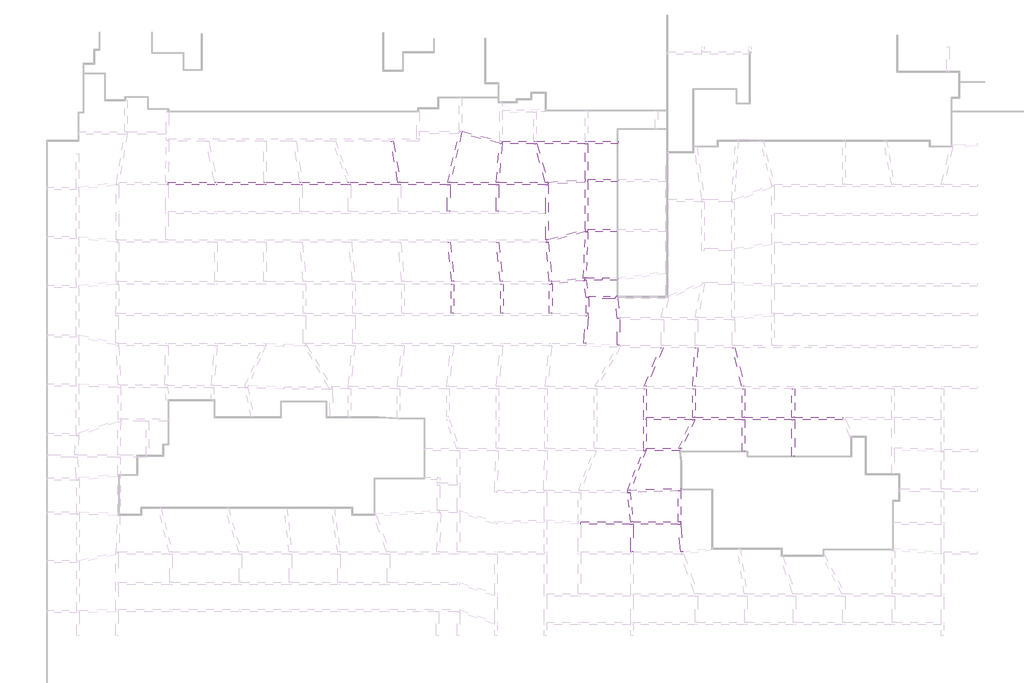
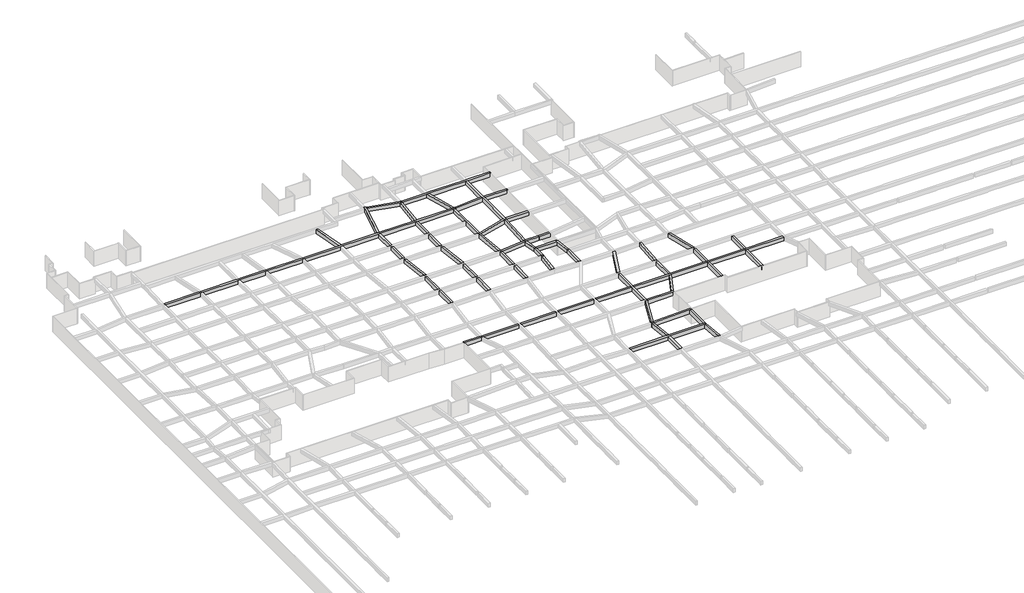
# One storey, part 37 of 45: 50 beams.
"""IFC4 building model written with IfcOpenShell, lengths in millimetres."""

from ifc_helpers import new_model, si_unit, frame, origin, place, context, project, spatial, polyline, outline, extrude, faceted_brep, element, save

model = new_model("IFC4")

# Units and contexts
model_context = context("Model", 3, world=origin())
ifc_project = project(units=[si_unit("LENGTHUNIT", "METRE", prefix="MILLI")], contexts=[model_context])

# Site, building, storey
site = spatial("IfcSite", under=ifc_project)
building = spatial("IfcBuilding", under=site)
storey = spatial("IfcBuildingStorey", under=building, Name="户型图", Elevation=0.0)

# Beams
placement = place(None, origin())
element("IfcBeam", 1, ObjectType="混凝土 - 矩形梁 : KL_beam", at=placement, inside=storey, context=model_context, shape_type="Brep", body=[
    faceted_brep([(-135857.1529868, 184740.2921988, 3300.0), (-135864.1350128, 184340.2921988, 3300.0), (-135860.6744654, 184340.2921988, 3300.0), (-128480.5216564, 184340.2921988, 3300.0), (-128080.5216564, 184340.2921988, 3300.0), (-120760.6744654, 184340.2921988, 3300.0), (-120360.6744654, 184340.2921988, 3300.0), (-115060.6744654, 184340.2921988, 3300.0), (-114660.6744654, 184340.2921988, 3300.0), (-107400.5216564, 184340.2921988, 3300.0), (-107000.5216564, 184340.2921988, 3300.0), (-99500.5216564, 184340.2921988, 3300.0), (-99100.5216564, 184340.2921988, 3300.0), (-91700.5216564, 184340.2921988, 3300.0), (-91300.5216564, 184340.2921988, 3300.0), (-83997.2475165, 184340.2921988, 3300.0), (-83597.2475165, 184340.2921988, 3300.0), (-76160.6744654, 184340.2921988, 3300.0), (-75760.6744654, 184340.2921988, 3300.0), (-75760.6744654, 184353.7891816, 3300.0), (-75760.6744654, 184568.4999459, 3300.0), (-75760.6744654, 184740.2921988, 3300.0), (-75810.1423565, 184740.2921988, 3300.0), (-76226.3954041, 184740.2921988, 3300.0), (-83579.0247125, 184740.2921988, 3300.0), (-83980.5526475, 184740.2921988, 3300.0), (-91248.9750891, 184740.2921988, 3300.0), (-91659.4967323, 184740.2921988, 3300.0), (-99132.7017302, 184740.2921988, 3300.0), (-99538.872375, 184740.2921988, 3300.0), (-107060.4801488, 184740.2921988, 3300.0), (-107486.1512578, 184740.2921988, 3300.0), (-114686.8171178, 184740.2921988, 3300.0), (-115090.7481468, 184740.2921988, 3300.0), (-120360.6744654, 184740.2921988, 3300.0), (-120760.6744654, 184740.2921988, 3300.0), (-128118.5648498, 184740.2921988, 3300.0), (-128527.5010878, 184740.2921988, 3300.0), (-135864.1350128, 184340.2921988, 2500.0), (-135860.6744654, 184340.2921988, 2500.0), (-128480.5216564, 184340.2921988, 2500.0), (-128080.5216564, 184340.2921988, 2500.0), (-120760.6744654, 184340.2921988, 2500.0), (-120360.6744654, 184340.2921988, 2500.0), (-115060.6744654, 184340.2921988, 2500.0), (-114660.6744654, 184340.2921988, 2500.0), (-107400.5216564, 184340.2921988, 2500.0), (-107000.5216564, 184340.2921988, 2500.0), (-99500.5216564, 184340.2921988, 2500.0), (-99100.5216564, 184340.2921988, 2500.0), (-91700.5216564, 184340.2921988, 2500.0), (-91300.5216564, 184340.2921988, 2500.0), (-83997.2475165, 184340.2921988, 2500.0), (-83597.2475165, 184340.2921988, 2500.0), (-76160.6744654, 184340.2921988, 2500.0), (-75760.6744654, 184340.2921988, 2500.0), (-135857.1529868, 184740.2921988, 2500.0), (-128527.5010878, 184740.2921988, 2500.0), (-128118.5648498, 184740.2921988, 2500.0), (-120760.6744654, 184740.2921988, 2500.0), (-120360.6744654, 184740.2921988, 2500.0), (-115090.7481468, 184740.2921988, 2500.0), (-114686.8171178, 184740.2921988, 2500.0), (-107486.1512578, 184740.2921988, 2500.0), (-107060.4801488, 184740.2921988, 2500.0), (-99538.872375, 184740.2921988, 2500.0), (-99132.7017302, 184740.2921988, 2500.0), (-91659.4967323, 184740.2921988, 2500.0), (-91248.9750891, 184740.2921988, 2500.0), (-83980.5526475, 184740.2921988, 2500.0), (-83579.0247125, 184740.2921988, 2500.0), (-76226.3954041, 184740.2921988, 2500.0), (-75810.1423565, 184740.2921988, 2500.0), (-75760.6744654, 184740.2921988, 2500.0), (-75760.6744654, 184568.4999459, 2500.0), (-75760.6744654, 184353.7891816, 2500.0)], [[[0, 1, 2, 3, 4, 5, 6, 7, 8, 9, 10, 11, 12, 13, 14, 15, 16, 17, 18, 19, 20, 21, 22, 23, 24, 25, 26, 27, 28, 29, 30, 31, 32, 33, 34, 35, 36, 37]], [[1, 38, 39, 40, 41, 42, 43, 44, 45, 46, 47, 48, 49, 50, 51, 52, 53, 54, 55, 18, 17, 16, 15, 14, 13, 12, 11, 10, 9, 8, 7, 6, 5, 4, 3, 2]], [[38, 56, 57, 58, 59, 60, 61, 62, 63, 64, 65, 66, 67, 68, 69, 70, 71, 72, 73, 74, 75, 55, 54, 53, 52, 51, 50, 49, 48, 47, 46, 45, 44, 43, 42, 41, 40, 39]], [[56, 0, 37, 36, 35, 34, 33, 32, 31, 30, 29, 28, 27, 26, 25, 24, 23, 22, 21, 73, 72, 71, 70, 69, 68, 67, 66, 65, 64, 63, 62, 61, 60, 59, 58, 57]], [[1, 0, 56, 38]], [[21, 20, 19, 18, 55, 75, 74, 73]]]),
])
element("IfcBeam", 2, ObjectType="混凝土 - 矩形梁 : KL_beam", at=placement, inside=storey, context=model_context, shape_type="SweptSolid", body=[
    extrude(outline(polyline([(-99132.7017302, 184740.2921988), (-99538.872375, 184740.2921988), (-100674.2344394, 191179.2504337), (-100268.0637947, 191179.2504337), (-99132.7017302, 184740.2921988)])), frame((0.0, 0.0, 2500.0), z_axis=(0.0, 0.0, 1.0), x_axis=(1.0, 0.0, 0.0)), (0.0, 0.0, 1.0), 800.0),
])
element("IfcBeam", 3, ObjectType="混凝土 - 矩形梁 : KL_beam", at=placement, inside=storey, context=model_context, shape_type="SweptSolid", body=[
    extrude(outline(polyline([(-91700.5216564, 184340.2921988), (-91300.5216564, 184340.2921988), (-91300.5216564, 180177.2946529), (-91700.5216564, 180177.2946529), (-91700.5216564, 184340.2921988)])), frame((0.0, 0.0, 2500.0), z_axis=(0.0, 0.0, 1.0), x_axis=(1.0, 0.0, 0.0)), (0.0, 0.0, 1.0), 800.0),
    extrude(outline(polyline([(-91300.5216564, 175615.3210168), (-91700.5216564, 175615.3210168), (-91700.5216564, 179777.2946529), (-91300.5216564, 179777.2946529), (-91300.5216564, 175615.3210168)])), frame((0.0, 0.0, 2500.0), z_axis=(0.0, 0.0, 1.0), x_axis=(1.0, 0.0, 0.0)), (0.0, 0.0, 1.0), 800.0),
])
element("IfcBeam", 4, ObjectType="混凝土 - 矩形梁 : KL_beam", at=placement, inside=storey, context=model_context, shape_type="Brep", body=[
    faceted_brep([(-89394.3421353, 192773.5900939, 3300.0), (-89784.0901613, 192863.5705156, 3300.0), (-89833.4279054, 192649.8652672, 3300.0), (-89884.7573746, 192427.5329095, 3300.0), (-91659.4967323, 184740.2921988, 3300.0), (-91248.9750891, 184740.2921988, 3300.0), (-89484.3362636, 192383.7826984, 3300.0), (-89394.3421353, 192773.5900939, 2500.0), (-91248.9750891, 184740.2921988, 2500.0), (-89484.3362636, 192383.7826984, 2500.0), (-89784.0901613, 192863.5705156, 2500.0), (-91659.4967323, 184740.2921988, 2500.0), (-89884.7573746, 192427.5329095, 2500.0), (-89833.4279054, 192649.8652672, 2500.0)], [[[0, 1, 2, 3, 4, 5, 6]], [[7, 0, 6, 5, 8, 9]], [[10, 7, 9, 8, 11, 12, 13]], [[1, 10, 13, 12, 11, 4, 3, 2]], [[5, 4, 11, 8]], [[1, 0, 7, 10]]]),
])
element("IfcBeam", 5, ObjectType="混凝土 - 矩形梁 : KL_beam", at=placement, inside=storey, context=model_context, shape_type="Brep", body=[
    faceted_brep([(-83050.6464251, 190779.68366, 3300.0), (-83046.2098772, 190830.3936346, 3300.0), (-83015.349565, 191183.1286161, 3300.0), (-83204.9191998, 191230.3936346, 3300.0), (-83429.5150082, 191286.3916589, 3300.0), (-89394.3421353, 192773.5900939, 3300.0), (-89484.3362636, 192383.7826984, 3300.0), (-83443.6026589, 190877.658653, 3300.0), (-83050.6464251, 190779.68366, 2500.0), (-89484.3362636, 192383.7826984, 2500.0), (-83443.6026589, 190877.658653, 2500.0), (-83015.349565, 191183.1286161, 2500.0), (-83046.2098772, 190830.3936346, 2500.0), (-89394.3421353, 192773.5900939, 2500.0), (-83429.5150082, 191286.3916589, 2500.0), (-83204.9191998, 191230.3936346, 2500.0), (-89782.5195472, 192870.3735927, 2500.0), (-89782.5195472, 192870.3735927, 3300.0), (-89433.4279054, 192783.3352708, 3300.0), (-89433.4279054, 192783.3352708, 2500.0), (-89784.0901613, 192863.5705156, 2500.0), (-89784.0901613, 192863.5705156, 3300.0)], [[[0, 1, 2, 3, 4, 5, 6, 7]], [[8, 0, 7, 6, 9, 10]], [[11, 12, 8, 10, 9, 13, 14, 15]], [[16, 17, 18, 5, 4, 3, 2, 11, 15, 14, 13, 19]], [[17, 16, 20, 21]], [[5, 13, 9, 6]], [[13, 5, 21, 20]], [[5, 18, 17, 21]], [[20, 16, 19, 13]], [[2, 1, 0, 8, 12, 11]]]),
])
element("IfcBeam", 6, ObjectType="混凝土 - 矩形梁 : KL_beam", at=placement, inside=storey, context=model_context, shape_type="SweptSolid", body=[
    extrude(outline(polyline([(-83443.6026589, 190877.658653), (-83050.6464251, 190779.68366), (-83579.0247125, 184740.2921988), (-83980.5526475, 184740.2921988), (-83443.6026589, 190877.658653)])), frame((0.0, 0.0, 2500.0), z_axis=(0.0, 0.0, 1.0), x_axis=(1.0, 0.0, 0.0)), (0.0, 0.0, 1.0), 800.0),
])
element("IfcBeam", 7, ObjectType="混凝土 - 矩形梁 : KL_beam", at=placement, inside=storey, context=model_context, shape_type="Brep", body=[
    faceted_brep([(-64729.476112, 191230.3936346, 3300.0), (-64729.476112, 190830.3936346, 3300.0), (-64729.476112, 190830.3936346, 2500.0), (-64729.476112, 191230.3936346, 2500.0), (-69489.476112, 191230.3936346, 3300.0), (-69889.476112, 191230.3936346, 3300.0), (-77629.5150082, 191230.3936346, 3300.0), (-78029.5150082, 191230.3936346, 3300.0), (-83029.5150082, 191230.3936346, 3300.0), (-83204.9191998, 191230.3936346, 3300.0), (-83015.349565, 191183.1286161, 3300.0), (-83046.2098772, 190830.3936346, 3300.0), (-77980.051169, 190830.3936346, 3300.0), (-77563.7981213, 190830.3936346, 3300.0), (-69889.476112, 190830.3936346, 3300.0), (-69489.476112, 190830.3936346, 3300.0), (-83046.2098772, 190830.3936346, 2500.0), (-77980.051169, 190830.3936346, 2500.0), (-77563.7981213, 190830.3936346, 2500.0), (-69889.476112, 190830.3936346, 2500.0), (-69489.476112, 190830.3936346, 2500.0), (-83015.349565, 191183.1286161, 2500.0), (-83204.9191998, 191230.3936346, 2500.0), (-83029.5150082, 191230.3936346, 2500.0), (-78029.5150082, 191230.3936346, 2500.0), (-77629.5150082, 191230.3936346, 2500.0), (-69889.476112, 191230.3936346, 2500.0), (-69489.476112, 191230.3936346, 2500.0)], [[[0, 1, 2, 3]], [[1, 0, 4, 5, 6, 7, 8, 9, 10, 11, 12, 13, 14, 15]], [[2, 1, 15, 14, 13, 12, 11, 16, 17, 18, 19, 20]], [[3, 2, 20, 19, 18, 17, 16, 21, 22, 23, 24, 25, 26, 27]], [[0, 3, 27, 26, 25, 24, 23, 22, 9, 8, 7, 6, 5, 4]], [[21, 10, 9, 22]], [[10, 21, 16, 11]]]),
])
element("IfcBeam", 8, ObjectType="混凝土 - 矩形梁 : KL_beam", at=placement, inside=storey, context=model_context, shape_type="Brep", body=[
    faceted_brep([(-69889.476112, 176868.8333665, 3300.0), (-69662.8012561, 176930.3936346, 3300.0), (-69489.476112, 176977.4652089, 3300.0), (-69489.476112, 177330.3936346, 3300.0), (-69489.476112, 184778.8171067, 3300.0), (-69489.476112, 185178.8171067, 3300.0), (-69489.476112, 190830.3936346, 3300.0), (-69889.476112, 190830.3936346, 3300.0), (-69889.476112, 185165.320124, 3300.0), (-69889.476112, 184764.3433647, 3300.0), (-69889.476112, 177283.3220602, 3300.0), (-69889.476112, 176868.8333665, 2500.0), (-69889.476112, 190830.3936346, 2500.0), (-69889.476112, 185165.320124, 2500.0), (-69889.476112, 184764.3433647, 2500.0), (-69889.476112, 177283.3220602, 2500.0), (-69489.476112, 176977.4652089, 2500.0), (-69662.8012561, 176930.3936346, 2500.0), (-69489.476112, 190830.3936346, 2500.0), (-69489.476112, 185178.8171067, 2500.0), (-69489.476112, 184778.8171067, 2500.0), (-69489.476112, 177330.3936346, 2500.0)], [[[0, 1, 2, 3, 4, 5, 6, 7, 8, 9, 10]], [[11, 0, 10, 9, 8, 7, 12, 13, 14, 15]], [[16, 17, 11, 15, 14, 13, 12, 18, 19, 20, 21]], [[2, 16, 21, 20, 19, 18, 6, 5, 4, 3]], [[7, 6, 18, 12]], [[2, 1, 0, 11, 17, 16]]]),
])
element("IfcBeam", 9, ObjectType="混凝土 - 矩形梁 : KL_beam", at=placement, inside=storey, context=model_context, shape_type="Brep", body=[
    faceted_brep([(-76031.325523, 175615.3210168, 3300.0), (-75977.9758113, 175215.3210168, 3300.0), (-75746.4906083, 175278.1876771, 3300.0), (-69900.6399035, 176865.8015084, 3300.0), (-69889.476112, 176868.8333665, 3300.0), (-69889.476112, 177283.3220602, 3300.0), (-75760.6744654, 175688.8243244, 3300.0), (-75977.9758113, 175215.3210168, 2500.0), (-75746.4906083, 175278.1876771, 2500.0), (-69900.6399035, 176865.8015084, 2500.0), (-69889.476112, 176868.8333665, 2500.0), (-76031.325523, 175615.3210168, 2500.0), (-75760.6744654, 175688.8243244, 2500.0), (-69889.476112, 177283.3220602, 2500.0)], [[[0, 1, 2, 3, 4, 5, 6]], [[1, 7, 8, 9, 10, 4, 3, 2]], [[7, 11, 12, 13, 10, 9, 8]], [[11, 0, 6, 5, 13, 12]], [[0, 11, 7, 1]], [[5, 4, 10, 13]]]),
])
element("IfcBeam", 10, ObjectType="混凝土 - 矩形梁 : KL_beam", at=placement, inside=storey, context=model_context, shape_type="Brep", body=[
    faceted_brep([(-64789.476112, 177330.3936346, 3300.0), (-69489.476112, 177330.3936346, 3300.0), (-69489.476112, 176977.4652089, 3300.0), (-69662.8012561, 176930.3936346, 3300.0), (-69497.7421026, 176930.3936346, 3300.0), (-64789.476112, 176930.3936346, 3300.0), (-69662.8012561, 176930.3936346, 2500.0), (-69497.7421026, 176930.3936346, 2500.0), (-64789.476112, 176930.3936346, 2500.0), (-69489.476112, 176977.4652089, 2500.0), (-69489.476112, 177330.3936346, 2500.0), (-64789.476112, 177330.3936346, 2500.0)], [[[0, 1, 2, 3, 4, 5]], [[5, 4, 3, 6, 7, 8]], [[8, 7, 6, 9, 10, 11]], [[1, 0, 11, 10]], [[9, 2, 1, 10]], [[2, 9, 6, 3]], [[0, 5, 8, 11]]]),
])
element("IfcBeam", 11, ObjectType="混凝土 - 矩形梁 : KL_beam", at=placement, inside=storey, context=model_context, shape_type="Brep", body=[
    faceted_brep([(-75760.6744654, 184340.2921988, 3300.0), (-76160.6744654, 184340.2921988, 3300.0), (-76160.6744654, 180177.2946529, 3300.0), (-76160.6744654, 179777.2946529, 3300.0), (-76160.6744654, 175615.3210168, 3300.0), (-76031.325523, 175615.3210168, 3300.0), (-75760.6744654, 175688.8243244, 3300.0), (-76160.6744654, 184340.2921988, 2500.0), (-76160.6744654, 180177.2946529, 2500.0), (-76160.6744654, 179777.2946529, 2500.0), (-76160.6744654, 175615.3210168, 2500.0), (-75760.6744654, 184340.2921988, 2500.0), (-75760.6744654, 175688.8243244, 2500.0), (-76031.325523, 175615.3210168, 2500.0)], [[[0, 1, 2, 3, 4, 5, 6]], [[1, 7, 8, 9, 10, 4, 3, 2]], [[7, 11, 12, 13, 10, 9, 8]], [[11, 0, 6, 12]], [[1, 0, 11, 7]], [[6, 5, 13, 12]], [[5, 4, 10, 13]]]),
])
element("IfcBeam", 12, ObjectType="混凝土 - 矩形梁 : KL_beam", at=placement, inside=storey, context=model_context, shape_type="Brep", body=[
    faceted_brep([(-75587.7690547, 169035.1135794, 3300.0), (-75186.161196, 169035.1135794, 3300.0), (-75187.9679462, 169055.2440151, 3300.0), (-75746.4906083, 175278.1876771, 3300.0), (-75760.6744654, 175274.3356308, 3300.0), (-75977.9758113, 175215.3210168, 3300.0), (-76142.4560482, 175215.3210168, 3300.0), (-75587.7690547, 169035.1135794, 2500.0), (-76142.4560482, 175215.3210168, 2500.0), (-75186.161196, 169035.1135794, 2500.0), (-75977.9758113, 175215.3210168, 2500.0), (-75760.6744654, 175274.3356308, 2500.0), (-75746.4906083, 175278.1876771, 2500.0), (-75187.9679462, 169055.2440151, 2500.0)], [[[0, 1, 2, 3, 4, 5, 6]], [[7, 0, 6, 8]], [[9, 7, 8, 10, 11, 12, 13]], [[1, 9, 13, 12, 3, 2]], [[1, 0, 7, 9]], [[3, 12, 11, 10, 5, 4]], [[6, 5, 10, 8]]]),
])
element("IfcBeam", 13, ObjectType="混凝土 - 矩形梁 : KL_beam", at=placement, inside=storey, context=model_context, shape_type="Brep", body=[
    faceted_brep([(-75186.161196, 169035.1135794, 3300.0), (-75186.161196, 168653.2306004, 3300.0), (-75169.0146925, 168655.0327706, 3300.0), (-70166.4570627, 169180.8227646, 3300.0), (-69988.1149016, 169199.5672811, 3300.0), (-70009.0780133, 169599.5672811, 3300.0), (-70191.535826, 169580.3901922, 3300.0), (-75187.9679462, 169055.2440151, 3300.0), (-75186.161196, 168653.2306004, 2500.0), (-75169.0146925, 168655.0327706, 2500.0), (-70166.4570627, 169180.8227646, 2500.0), (-69988.1149016, 169199.5672811, 2500.0), (-75186.161196, 169035.1135794, 2500.0), (-75187.9679462, 169055.2440151, 2500.0), (-70191.535826, 169580.3901922, 2500.0), (-70009.0780133, 169599.5672811, 2500.0)], [[[0, 1, 2, 3, 4, 5, 6, 7]], [[1, 8, 9, 10, 11, 4, 3, 2]], [[8, 12, 13, 14, 15, 11, 10, 9]], [[5, 15, 14, 13, 7, 6]], [[1, 0, 12, 8]], [[0, 7, 13, 12]], [[5, 4, 11, 15]]]),
    faceted_brep([(-75569.0146925, 168612.9910764, 2500.0), (-75569.0146925, 168612.9910764, 3300.0), (-75569.0146925, 168635.1135794, 3300.0), (-75569.0146925, 168635.1135794, 2500.0), (-75358.5331366, 168635.1135794, 3300.0), (-75358.5331366, 168635.1135794, 2500.0), (-75551.868189, 168635.1135794, 2500.0), (-75551.868189, 168635.1135794, 3300.0)], [[[0, 1, 2, 3]], [[4, 5, 6, 3, 2, 7]], [[1, 4, 7, 2]], [[1, 0, 5, 4]], [[5, 0, 3, 6]]]),
])
element("IfcBeam", 14, ObjectType="混凝土 - 矩形梁 : KL_beam", at=placement, inside=storey, context=model_context, shape_type="Brep", body=[
    faceted_brep([(-67198.5964575, 169599.5672811, 3300.0), (-69790.4513817, 169599.5672811, 3300.0), (-70009.0780133, 169599.5672811, 3300.0), (-69988.1149016, 169199.5672811, 3300.0), (-69764.4398522, 169199.5672811, 3300.0), (-67198.5964575, 169199.5672811, 3300.0), (-69988.1149016, 169199.5672811, 2500.0), (-69764.4398522, 169199.5672811, 2500.0), (-67198.5964575, 169199.5672811, 2500.0), (-70009.0780133, 169599.5672811, 2500.0), (-69790.4513817, 169599.5672811, 2500.0), (-67198.5964575, 169599.5672811, 2500.0)], [[[0, 1, 2, 3, 4, 5]], [[5, 4, 3, 6, 7, 8]], [[8, 7, 6, 9, 10, 11]], [[2, 1, 0, 11, 10, 9]], [[2, 9, 6, 3]], [[0, 5, 8, 11]]]),
])
element("IfcBeam", 15, ObjectType="混凝土 - 矩形梁 : KL_beam", at=placement, inside=storey, context=model_context, shape_type="Brep", body=[
    faceted_brep([(-70191.535826, 169580.3901922, 3300.0), (-70009.0780133, 169599.5672811, 3300.0), (-69790.4513817, 169599.5672811, 3300.0), (-69497.7421026, 176930.3936346, 3300.0), (-69662.8012561, 176930.3936346, 3300.0), (-69889.476112, 176868.8333665, 3300.0), (-69900.6399035, 176865.8015084, 3300.0), (-70191.535826, 169580.3901922, 2500.0), (-69900.6399035, 176865.8015084, 2500.0), (-70009.0780133, 169599.5672811, 2500.0), (-69889.476112, 176868.8333665, 2500.0), (-69662.8012561, 176930.3936346, 2500.0), (-69497.7421026, 176930.3936346, 2500.0), (-69790.4513817, 169599.5672811, 2500.0)], [[[0, 1, 2, 3, 4, 5, 6]], [[7, 0, 6, 8]], [[9, 7, 8, 10, 11, 12, 13]], [[2, 13, 12, 3]], [[1, 0, 7, 9]], [[2, 1, 9, 13]], [[8, 6, 5, 4, 11, 10]], [[4, 3, 12, 11]]]),
])
element("IfcBeam", 16, ObjectType="混凝土 - 矩形梁 : KL_beam", at=placement, inside=storey, context=model_context, shape_type="SweptSolid", body=[
    extrude(outline(polyline([(-83997.2475165, 184340.2921988), (-83597.2475165, 184340.2921988), (-83597.2475165, 180177.2946529), (-83997.2475165, 180177.2946529), (-83997.2475165, 184340.2921988)])), frame((0.0, 0.0, 2500.0), z_axis=(0.0, 0.0, 1.0), x_axis=(1.0, 0.0, 0.0)), (0.0, 0.0, 1.0), 800.0),
    extrude(outline(polyline([(-83597.2475165, 175615.3210168), (-83997.2475165, 175615.3210168), (-83997.2475165, 179777.2946529), (-83597.2475165, 179777.2946529), (-83597.2475165, 175615.3210168)])), frame((0.0, 0.0, 2500.0), z_axis=(0.0, 0.0, 1.0), x_axis=(1.0, 0.0, 0.0)), (0.0, 0.0, 1.0), 800.0),
])
element("IfcBeam", 17, ObjectType="混凝土 - 矩形梁 : KL_beam", at=placement, inside=storey, context=model_context, shape_type="SweptSolid", body=[
    extrude(outline(polyline([(-91680.6024653, 175215.3210168), (-91278.3991535, 175215.3210168), (-90628.833177, 169035.1135794), (-91031.0364888, 169035.1135794), (-91680.6024653, 175215.3210168)])), frame((0.0, 0.0, 2500.0), z_axis=(0.0, 0.0, 1.0), x_axis=(1.0, 0.0, 0.0)), (0.0, 0.0, 1.0), 800.0),
])
element("IfcBeam", 18, ObjectType="混凝土 - 矩形梁 : KL_beam", at=placement, inside=storey, context=model_context, shape_type="SweptSolid", body=[
    extrude(outline(polyline([(-83977.3283253, 175215.3210168), (-83575.1250135, 175215.3210168), (-82925.559037, 169035.1135794), (-83327.7623488, 169035.1135794), (-83977.3283253, 175215.3210168)])), frame((0.0, 0.0, 2500.0), z_axis=(0.0, 0.0, 1.0), x_axis=(1.0, 0.0, 0.0)), (0.0, 0.0, 1.0), 800.0),
])
element("IfcBeam", 19, ObjectType="混凝土 - 矩形梁 : KL_beam", at=placement, inside=storey, context=model_context, shape_type="SweptSolid", body=[
    extrude(outline(polyline([(-90724.7994609, 159263.2495721), (-91124.7994609, 159263.2495721), (-91124.7994609, 163650.6823883), (-90724.7994609, 163650.6823883), (-90724.7994609, 159263.2495721)])), frame((0.0, 0.0, 2500.0), z_axis=(0.0, 0.0, 1.0), x_axis=(1.0, 0.0, 0.0)), (0.0, 0.0, 1.0), 800.0),
    extrude(outline(polyline([(-91124.7994609, 168635.1135794), (-90724.7994609, 168635.1135794), (-90724.7994609, 164050.6823883), (-91124.7994609, 164050.6823883), (-91124.7994609, 168635.1135794)])), frame((0.0, 0.0, 2500.0), z_axis=(0.0, 0.0, 1.0), x_axis=(1.0, 0.0, 0.0)), (0.0, 0.0, 1.0), 800.0),
])
element("IfcBeam", 20, ObjectType="混凝土 - 矩形梁 : KL_beam", at=placement, inside=storey, context=model_context, shape_type="SweptSolid", body=[
    extrude(outline(polyline([(-83305.6398459, 168635.1135794), (-82905.6398459, 168635.1135794), (-82905.6398459, 164050.6823883), (-83305.6398459, 164050.6823883), (-83305.6398459, 168635.1135794)])), frame((0.0, 0.0, 2500.0), z_axis=(0.0, 0.0, 1.0), x_axis=(1.0, 0.0, 0.0)), (0.0, 0.0, 1.0), 800.0),
    extrude(outline(polyline([(-82905.6398459, 159263.2495721), (-83305.6398459, 159263.2495721), (-83305.6398459, 163650.6823883), (-82905.6398459, 163650.6823883), (-82905.6398459, 159263.2495721)])), frame((0.0, 0.0, 2500.0), z_axis=(0.0, 0.0, 1.0), x_axis=(1.0, 0.0, 0.0)), (0.0, 0.0, 1.0), 800.0),
])
element("IfcBeam", 21, ObjectType="混凝土 - 矩形梁 : KL_beam", at=placement, inside=storey, context=model_context, shape_type="SweptSolid", body=[
    extrude(outline(polyline([(-75358.5331366, 168635.1135794), (-75186.161196, 168635.1135794), (-75186.161196, 168653.2306004), (-75169.0146925, 168655.0327706), (-75169.0146925, 164050.6823883), (-75569.0146925, 164050.6823883), (-75569.0146925, 168612.9910764), (-75358.5331366, 168635.1135794)])), frame((0.0, 0.0, 2500.0), z_axis=(0.0, 0.0, 1.0), x_axis=(1.0, 0.0, 0.0)), (0.0, 0.0, 1.0), 800.0),
    extrude(outline(polyline([(-75169.0146925, 159263.2495721), (-75569.0146925, 159263.2495721), (-75569.0146925, 163650.6823883), (-75169.0146925, 163650.6823883), (-75169.0146925, 159263.2495721)])), frame((0.0, 0.0, 2500.0), z_axis=(0.0, 0.0, 1.0), x_axis=(1.0, 0.0, 0.0)), (0.0, 0.0, 1.0), 800.0),
])
element("IfcBeam", 22, ObjectType="混凝土 - 矩形梁 : KL_beam", at=placement, inside=storey, context=model_context, shape_type="SweptSolid", body=[
    extrude(outline(polyline([(-69845.6243611, 163650.6823883), (-69444.6043733, 163650.6823883), (-69758.1275482, 159263.2495721), (-70159.147536, 159263.2495721), (-69845.6243611, 163650.6823883)])), frame((0.0, 0.0, 2500.0), z_axis=(0.0, 0.0, 1.0), x_axis=(1.0, 0.0, 0.0)), (0.0, 0.0, 1.0), 800.0),
])
element("IfcBeam", 23, ObjectType="混凝土 - 矩形梁 : KL_beam", at=placement, inside=storey, context=model_context, shape_type="Brep", body=[
    faceted_brep([(-70166.4570627, 169180.8227646, 3300.0), (-69744.9443936, 166519.4965113, 3300.0), (-69344.9443936, 166550.977194, 3300.0), (-69374.1282565, 166735.2368527, 3300.0), (-69764.4398522, 169199.5672811, 3300.0), (-69988.1149016, 169199.5672811, 3300.0), (-70166.4570627, 169180.8227646, 2500.0), (-69744.9443936, 166519.4965113, 2500.0), (-69988.1149016, 169199.5672811, 2500.0), (-69764.4398522, 169199.5672811, 2500.0), (-69374.1282565, 166735.2368527, 2500.0), (-69344.9443936, 166550.977194, 2500.0)], [[[0, 1, 2, 3, 4, 5]], [[1, 0, 6, 7]], [[7, 6, 8, 9, 10, 11]], [[2, 11, 10, 9, 4, 3]], [[0, 5, 8, 6]], [[5, 4, 9, 8]], [[2, 1, 7, 11]]]),
])
element("IfcBeam", 24, ObjectType="混凝土 - 矩形梁 : KL_beam", at=placement, inside=storey, context=model_context, shape_type="Brep", body=[
    faceted_brep([(-60687.7540188, 142284.531219, 3300.0), (-60350.0447554, 142284.531219, 3300.0), (-60287.7540188, 142284.531219, 3300.0), (-60287.7540188, 142447.6410632, 3300.0), (-60287.7540188, 142684.531219, 3300.0), (-60287.7540188, 147179.5060773, 3300.0), (-60287.7540188, 147579.5060773, 3300.0), (-60287.7540188, 152079.7935386, 3300.0), (-60687.7540188, 152079.7935386, 3300.0), (-60687.7540188, 147579.5060773, 3300.0), (-60687.7540188, 147179.5060773, 3300.0), (-60687.7540188, 142684.531219, 3300.0), (-60687.7540188, 142284.531219, 2500.0), (-60687.7540188, 152079.7935386, 2500.0), (-60687.7540188, 147579.5060773, 2500.0), (-60687.7540188, 147179.5060773, 2500.0), (-60687.7540188, 142684.531219, 2500.0), (-60287.7540188, 142284.531219, 2500.0), (-60350.0447554, 142284.531219, 2500.0), (-60287.7540188, 152079.7935386, 2500.0), (-60287.7540188, 147579.5060773, 2500.0), (-60287.7540188, 147179.5060773, 2500.0), (-60287.7540188, 142684.531219, 2500.0), (-60287.7540188, 142447.6410632, 2500.0)], [[[0, 1, 2, 3, 4, 5, 6, 7, 8, 9, 10, 11]], [[12, 0, 11, 10, 9, 8, 13, 14, 15, 16]], [[17, 18, 12, 16, 15, 14, 13, 19, 20, 21, 22, 23]], [[2, 17, 23, 22, 21, 20, 19, 7, 6, 5, 4, 3]], [[8, 7, 19, 13]], [[2, 1, 0, 12, 18, 17]]]),
])
element("IfcBeam", 25, ObjectType="混凝土 - 矩形梁 : KL_beam", at=placement, inside=storey, context=model_context, shape_type="SweptSolid", body=[
    extrude(outline(polyline([(-60185.5869801, 152479.7935386), (-60620.131131, 152479.7935386), (-58031.4610211, 158578.3181414), (-57596.9168701, 158578.3181414), (-60185.5869801, 152479.7935386)])), frame((0.0, 0.0, 2500.0), z_axis=(0.0, 0.0, 1.0), x_axis=(1.0, 0.0, 0.0)), (0.0, 0.0, 1.0), 800.0),
])
element("IfcBeam", 26, ObjectType="混凝土 - 矩形梁 : KL_beam", at=placement, inside=storey, context=model_context, shape_type="SweptSolid", body=[
    extrude(outline(polyline([(-52476.9979937, 152479.7935386), (-52877.5469321, 152479.7935386), (-52557.9368008, 158578.3181414), (-52157.3878624, 158578.3181414), (-52476.9979937, 152479.7935386)])), frame((0.0, 0.0, 2500.0), z_axis=(0.0, 0.0, 1.0), x_axis=(1.0, 0.0, 0.0)), (0.0, 0.0, 1.0), 800.0),
])
element("IfcBeam", 27, ObjectType="混凝土 - 矩形梁 : KL_beam", at=placement, inside=storey, context=model_context, shape_type="Brep", body=[
    faceted_brep([(-45143.7423452, 152479.7935386, 3300.0), (-44731.4968935, 152479.7935386, 3300.0), (-46244.2344007, 158547.0522899, 3300.0), (-46252.029853, 158578.3181414, 3300.0), (-46664.2753047, 158578.3181414, 3300.0), (-44731.4968935, 152479.7935386, 2500.0), (-46244.2344007, 158547.0522899, 2500.0), (-46252.029853, 158578.3181414, 2500.0), (-45143.7423452, 152479.7935386, 2500.0), (-46664.2753047, 158578.3181414, 2500.0)], [[[0, 1, 2, 3, 4]], [[1, 5, 6, 7, 3, 2]], [[5, 8, 9, 7, 6]], [[8, 0, 4, 9]], [[1, 0, 8, 5]], [[4, 3, 7, 9]]]),
])
element("IfcBeam", 28, ObjectType="混凝土 - 矩形梁 : KL_beam", at=placement, inside=storey, context=model_context, shape_type="Brep", body=[
    faceted_brep([(-64844.2344007, 163189.8806768, 3300.0), (-64844.2344007, 158994.7405249, 3300.0), (-64647.7624548, 158984.4438666, 3300.0), (-64637.1523876, 158978.3181414, 3300.0), (-64444.2344007, 158978.3181414, 3300.0), (-64444.2344007, 163000.3622326, 3300.0), (-64444.2344007, 163210.8437885, 3300.0), (-64844.2344007, 163189.8806768, 2500.0), (-64844.2344007, 158994.7405249, 2500.0), (-64444.2344007, 163210.8437885, 2500.0), (-64444.2344007, 163000.3622326, 2500.0), (-64444.2344007, 158978.3181414, 2500.0), (-64637.1523876, 158978.3181414, 2500.0), (-64647.7624548, 158984.4438666, 2500.0)], [[[0, 1, 2, 3, 4, 5, 6]], [[1, 0, 7, 8]], [[8, 7, 9, 10, 11, 12, 13]], [[9, 6, 5, 4, 11, 10]], [[13, 2, 1, 8]], [[2, 13, 12, 3]], [[4, 3, 12, 11]], [[6, 9, 7, 0]]]),
])
element("IfcBeam", 29, ObjectType="混凝土 - 矩形梁 : KL_beam", at=placement, inside=storey, context=model_context, shape_type="Brep", body=[
    faceted_brep([(-65206.9062787, 166640.473102, 3300.0), (-65174.8246562, 166335.2368527, 3300.0), (-64844.2344007, 163189.8806768, 3300.0), (-64444.2344007, 163210.8437885, 3300.0), (-64464.1535918, 163400.3622326, 3300.0), (-64767.0558265, 166282.2844873, 3300.0), (-64809.0975206, 166682.2844873, 3300.0), (-64444.2344007, 163210.8437885, 2500.0), (-64464.1535918, 163400.3622326, 2500.0), (-64767.0558265, 166282.2844873, 2500.0), (-64809.0975206, 166682.2844873, 2500.0), (-64844.2344007, 163189.8806768, 2500.0), (-65174.8246562, 166335.2368527, 2500.0), (-65206.9062787, 166640.473102, 2500.0)], [[[0, 1, 2, 3, 4, 5, 6]], [[6, 5, 4, 3, 7, 8, 9, 10]], [[10, 9, 8, 7, 11, 12, 13]], [[2, 1, 0, 13, 12, 11]], [[2, 11, 7, 3]], [[0, 6, 10, 13]]]),
])
element("IfcBeam", 30, ObjectType="混凝土 - 矩形梁 : KL_beam", at=placement, inside=storey, context=model_context, shape_type="Brep", body=[
    faceted_brep([(-77563.7981213, 190830.3936346, 3300.0), (-77980.051169, 190830.3936346, 3300.0), (-76226.3954041, 184740.2921988, 3300.0), (-75810.1423565, 184740.2921988, 3300.0), (-75813.2514305, 184751.0894013, 3300.0), (-77563.7981213, 190830.3936346, 2500.0), (-75810.1423565, 184740.2921988, 2500.0), (-75813.2514305, 184751.0894013, 2500.0), (-77980.051169, 190830.3936346, 2500.0), (-76226.3954041, 184740.2921988, 2500.0)], [[[0, 1, 2, 3, 4]], [[5, 0, 4, 3, 6, 7]], [[8, 5, 7, 6, 9]], [[1, 8, 9, 2]], [[1, 0, 5, 8]], [[2, 9, 6, 3]]]),
    faceted_brep([(-75760.6744654, 184353.7891816, 3300.0), (-75760.6744654, 184568.4999459, 3300.0), (-75760.6744654, 184568.4999459, 2500.0), (-75760.6744654, 184353.7891816, 2500.0), (-75700.0684467, 184358.0271673, 2500.0), (-75700.0684467, 184358.0271673, 3300.0)], [[[0, 1, 2, 3]], [[4, 5, 0, 3]], [[5, 1, 0]], [[1, 5, 4, 2]], [[2, 4, 3]]]),
])
element("IfcBeam", 31, ObjectType="混凝土 - 矩形梁 : KL_beam", at=placement, inside=storey, context=model_context, shape_type="SweptSolid", body=[
    extrude(outline(polyline([(-69889.476112, 185165.320124), (-69889.476112, 184764.3433647), (-75700.0684467, 184358.0271673), (-75760.6744654, 184568.4999459), (-75760.6744654, 184740.2921988), (-75810.1423565, 184740.2921988), (-75813.2514305, 184751.0894013), (-69889.476112, 185165.320124)])), frame((0.0, 0.0, 2500.0), z_axis=(0.0, 0.0, 1.0), x_axis=(1.0, 0.0, 0.0)), (0.0, 0.0, 1.0), 800.0),
])
element("IfcBeam", 32, ObjectType="混凝土 - 矩形梁 : KL_beam", at=placement, inside=storey, context=model_context, shape_type="SweptSolid", body=[
    extrude(outline(polyline([(-64689.476112, 185178.8171067), (-64689.476112, 184778.8171067), (-69489.476112, 184778.8171067), (-69489.476112, 185178.8171067), (-64689.476112, 185178.8171067)])), frame((0.0, 0.0, 2500.0), z_axis=(0.0, 0.0, 1.0), x_axis=(1.0, 0.0, 0.0)), (0.0, 0.0, 1.0), 800.0),
])
element("IfcBeam", 33, ObjectType="混凝土 - 矩形梁 : KL_beam", at=placement, inside=storey, context=model_context, shape_type="SweptSolid", body=[
    extrude(outline(polyline([(-64812.5818199, 169599.5672811), (-64784.6110951, 169199.5672811), (-67198.5964575, 169199.5672811), (-67198.5964575, 169599.5672811), (-64812.5818199, 169599.5672811)])), frame((0.0, 0.0, 2500.0), z_axis=(0.0, 0.0, 1.0), x_axis=(1.0, 0.0, 0.0)), (0.0, 0.0, 1.0), 800.0),
])
element("IfcBeam", 34, ObjectType="混凝土 - 矩形梁 : KL_beam", at=placement, inside=storey, context=model_context, shape_type="Brep", body=[
    faceted_brep([(-69344.9443936, 163735.2368527, 2500.0), (-69344.9443936, 163735.2368527, 3300.0), (-69444.6043733, 163735.2368527, 3300.0), (-69444.6043733, 163735.2368527, 2500.0), (-69344.9443936, 166335.2368527, 3300.0), (-69344.9443936, 166550.977194, 3300.0), (-69744.9443936, 166519.4965113, 3300.0), (-69744.9443936, 164050.6823883, 3300.0), (-69444.6043733, 164050.6823883, 3300.0), (-69744.9443936, 166519.4965113, 2500.0), (-69744.9443936, 164050.6823883, 2500.0), (-69344.9443936, 166550.977194, 2500.0), (-69344.9443936, 166335.2368527, 2500.0), (-69444.6043733, 164050.6823883, 2500.0)], [[[0, 1, 2, 3]], [[1, 4, 5, 6, 7, 8, 2]], [[6, 9, 10, 7]], [[11, 12, 0, 3, 13, 10, 9]], [[1, 0, 12, 11, 5, 4]], [[5, 11, 9, 6]], [[13, 8, 7, 10]], [[8, 13, 3, 2]]]),
])
element("IfcBeam", 35, ObjectType="混凝土 - 矩形梁 : KL_beam", at=placement, inside=storey, context=model_context, shape_type="SweptSolid", body=[
    extrude(outline(polyline([(-69374.1282565, 166735.2368527), (-64814.6630385, 166735.2368527), (-64809.0975206, 166682.2844873), (-65206.9062787, 166640.473102), (-65174.8246562, 166335.2368527), (-69344.9443936, 166335.2368527), (-69344.9443936, 166550.977194), (-69374.1282565, 166735.2368527)])), frame((0.0, 0.0, 2500.0), z_axis=(0.0, 0.0, 1.0), x_axis=(1.0, 0.0, 0.0)), (0.0, 0.0, 1.0), 800.0),
])
element("IfcBeam", 36, ObjectType="混凝土 - 矩形梁 : KL_beam", at=placement, inside=storey, context=model_context, shape_type="Brep", body=[
    faceted_brep([(-60287.7540188, 142447.6410632, 3300.0), (-60197.286994, 142684.531219, 3300.0), (-60287.7540188, 142684.531219, 3300.0), (-60287.7540188, 142447.6410632, 2500.0), (-60197.286994, 142684.531219, 2500.0), (-60287.7540188, 142684.531219, 2500.0)], [[[0, 1, 2]], [[1, 0, 3, 4]], [[4, 3, 5]], [[5, 2, 1, 4]], [[0, 2, 5, 3]]]),
    faceted_brep([(-60778.2210435, 142284.531219, 3300.0), (-60778.2210435, 142284.531219, 2500.0), (-63157.3471554, 136054.7302845, 2500.0), (-63157.3471554, 136054.7302845, 3300.0), (-60687.7540188, 142284.531219, 3300.0), (-60350.0447554, 142284.531219, 3300.0), (-60350.0447554, 142284.531219, 2500.0), (-60687.7540188, 142284.531219, 2500.0), (-62729.1708674, 136054.7302845, 2500.0), (-62729.1708674, 136054.7302845, 3300.0)], [[[0, 1, 2, 3]], [[1, 0, 4, 5, 6, 7]], [[3, 2, 8, 9]], [[5, 4, 0, 3, 9]], [[6, 5, 9, 8]], [[1, 7, 6, 8, 2]]]),
])
element("IfcBeam", 37, ObjectType="混凝土 - 矩形梁 : KL_beam", at=placement, inside=storey, context=model_context, shape_type="Brep", body=[
    faceted_brep([(-54819.6378921, 135940.8706076, 3300.0), (-54833.5976908, 136340.6269384, 3300.0), (-63159.1953807, 136049.8906606, 3300.0), (-63223.286158, 135882.0673651, 3300.0), (-63200.5257506, 135648.2035546, 3300.0), (-63013.6246592, 135654.7302845, 3300.0), (-62880.1485856, 135659.3913717, 3300.0), (-62799.9970878, 135662.1903237, 3300.0), (-55219.6378921, 135926.9022998, 3300.0), (-54819.6378921, 135940.8706076, 2500.0), (-63200.5257506, 135648.2035546, 2500.0), (-63013.6246592, 135654.7302845, 2500.0), (-62880.1485856, 135659.3913717, 2500.0), (-62799.9970878, 135662.1903237, 2500.0), (-55219.6378921, 135926.9022998, 2500.0), (-54833.5976908, 136340.6269384, 2500.0), (-63223.286158, 135882.0673651, 2500.0), (-63159.1953807, 136049.8906606, 2500.0)], [[[0, 1, 2, 3, 4, 5, 6, 7, 8]], [[9, 0, 8, 7, 6, 5, 4, 10, 11, 12, 13, 14]], [[15, 9, 14, 13, 12, 11, 10, 16, 17]], [[1, 15, 17, 2]], [[3, 16, 10, 4]], [[16, 3, 2, 17]], [[1, 0, 9, 15]]]),
])
element("IfcBeam", 38, ObjectType="混凝土 - 矩形梁 : KL_beam", at=placement, inside=storey, context=model_context, shape_type="SweptSolid", body=[
    extrude(outline(polyline([(-63200.5257506, 135648.2035546), (-63013.6246592, 135654.7302845), (-62881.9286288, 135654.7302845), (-62880.1485856, 135659.3913717), (-62799.9970878, 135662.1903237), (-62351.5836814, 131054.7302845), (-62753.4735833, 131054.7302845), (-63200.5257506, 135648.2035546)])), frame((0.0, 0.0, 2500.0), z_axis=(0.0, 0.0, 1.0), x_axis=(1.0, 0.0, 0.0)), (0.0, 0.0, 1.0), 800.0),
])
element("IfcBeam", 39, ObjectType="混凝土 - 矩形梁 : KL_beam", at=placement, inside=storey, context=model_context, shape_type="Brep", body=[
    faceted_brep([(-54802.7541897, 130654.7302845, 3300.0), (-54819.6378921, 130862.8302425, 3300.0), (-54835.2072523, 131054.7302845, 3300.0), (-55219.6378921, 131054.7302845, 3300.0), (-62351.5836814, 131054.7302845, 3300.0), (-62753.4735833, 131054.7302845, 3300.0), (-70619.6378921, 131054.7302845, 3300.0), (-70619.6378921, 130654.7302845, 3300.0), (-62733.0898312, 130654.7302845, 3300.0), (-62333.0898312, 130654.7302845, 3300.0), (-55204.0685319, 130654.7302845, 3300.0), (-54802.7541897, 130654.7302845, 2500.0), (-70619.6378921, 130654.7302845, 2500.0), (-62733.0898312, 130654.7302845, 2500.0), (-62333.0898312, 130654.7302845, 2500.0), (-55204.0685319, 130654.7302845, 2500.0), (-54835.2072523, 131054.7302845, 2500.0), (-54819.6378921, 130862.8302425, 2500.0), (-70619.6378921, 131054.7302845, 2500.0), (-62753.4735833, 131054.7302845, 2500.0), (-62351.5836814, 131054.7302845, 2500.0), (-55219.6378921, 131054.7302845, 2500.0)], [[[0, 1, 2, 3, 4, 5, 6, 7, 8, 9, 10]], [[11, 0, 10, 9, 8, 7, 12, 13, 14, 15]], [[16, 17, 11, 15, 14, 13, 12, 18, 19, 20, 21]], [[2, 16, 21, 20, 19, 18, 6, 5, 4, 3]], [[7, 6, 18, 12]], [[2, 1, 0, 11, 17, 16]]]),
])
element("IfcBeam", 40, ObjectType="混凝土 - 矩形梁 : KL_beam", at=placement, inside=storey, context=model_context, shape_type="Brep", body=[
    faceted_brep([(-62733.0898312, 126289.9393475, 3300.0), (-62729.0040152, 126289.9393475, 3300.0), (-62333.0898312, 126289.9393475, 3300.0), (-62333.0898312, 126290.334816, 3300.0), (-62333.0898312, 130654.7302845, 3300.0), (-62733.0898312, 130654.7302845, 3300.0), (-62733.0898312, 126289.9393475, 2500.0), (-62733.0898312, 130654.7302845, 2500.0), (-62333.0898312, 126289.9393475, 2500.0), (-62729.0040152, 126289.9393475, 2500.0), (-62333.0898312, 130654.7302845, 2500.0), (-62333.0898312, 126290.334816, 2500.0)], [[[0, 1, 2, 3, 4, 5]], [[6, 0, 5, 7]], [[8, 9, 6, 7, 10, 11]], [[2, 8, 11, 10, 4, 3]], [[8, 2, 1, 0, 6, 9]], [[5, 4, 10, 7]]]),
])
element("IfcBeam", 41, ObjectType="混凝土 - 矩形梁 : KL_beam", at=placement, inside=storey, context=model_context, shape_type="SweptSolid", body=[
    extrude(outline(polyline([(-55204.0685319, 130654.7302845), (-54802.7541897, 130654.7302845), (-54450.8961138, 126317.9059876), (-54647.0751936, 126290.334816), (-54849.9735336, 126290.334816), (-55204.0685319, 130654.7302845)])), frame((0.0, 0.0, 2500.0), z_axis=(0.0, 0.0, 1.0), x_axis=(1.0, 0.0, 0.0)), (0.0, 0.0, 1.0), 800.0),
])
element("IfcBeam", 42, ObjectType="混凝土 - 矩形梁 : KL_beam", at=placement, inside=storey, context=model_context, shape_type="Brep", body=[
    faceted_brep([(-54819.6378921, 135940.8706076, 3300.0), (-55219.6378921, 135926.9022998, 3300.0), (-55219.6378921, 131054.7302845, 3300.0), (-54835.2072523, 131054.7302845, 3300.0), (-54819.6378921, 130862.8302425, 3300.0), (-54819.6378921, 136341.1144253, 2500.0), (-54819.6378921, 136341.1144253, 3300.0), (-54819.6378921, 130862.8302425, 2500.0), (-54819.6378921, 135940.8706076, 2500.0), (-55219.6378921, 135926.9022998, 2500.0), (-54835.2072523, 131054.7302845, 2500.0), (-55219.6378921, 131054.7302845, 2500.0), (-54833.5976908, 136340.6269384, 2500.0), (-54833.5976908, 136340.6269384, 3300.0)], [[[0, 1, 2, 3, 4]], [[5, 6, 0, 4, 7, 8]], [[9, 8, 7, 10, 11]], [[1, 9, 11, 2]], [[6, 5, 12, 13]], [[0, 8, 9, 1]], [[8, 0, 13, 12]], [[6, 13, 0]], [[12, 5, 8]], [[10, 3, 2, 11]], [[3, 10, 7, 4]]]),
])
element("IfcBeam", 43, ObjectType="混凝土 - 矩形梁 : KL_beam", at=placement, inside=storey, context=model_context, shape_type="Brep", body=[
    faceted_brep([(-95343.1220374, 147579.5060773, 3300.0), (-95343.1220374, 147579.5060773, 2500.0), (-95343.1220374, 147179.5060773, 2500.0), (-95343.1220374, 147179.5060773, 3300.0), (-84024.3638582, 147579.5060773, 3300.0), (-84024.3638582, 147179.5060773, 3300.0), (-84024.3638582, 147179.5060773, 2500.0), (-84024.3638582, 147579.5060773, 2500.0), (-91855.4844058, 147179.5060773, 3300.0), (-91431.3906383, 147179.5060773, 3300.0), (-91443.5387872, 147579.5060773, 3300.0), (-91843.5387872, 147579.5060773, 3300.0), (-91855.4844058, 147179.5060773, 2500.0), (-91431.3906383, 147179.5060773, 2500.0), (-91843.5387872, 147579.5060773, 2500.0), (-91443.5387872, 147579.5060773, 2500.0)], [[[0, 1, 2, 3]], [[4, 5, 6, 7]], [[0, 3, 8, 9, 5, 4, 10, 11]], [[3, 2, 12, 13, 6, 5, 9, 8]], [[2, 1, 14, 15, 7, 6, 13, 12]], [[1, 0, 11, 10, 4, 7, 15, 14]]]),
    faceted_brep([(-83624.3638582, 147579.5060773, 3300.0), (-83624.3638582, 147179.5060773, 3300.0), (-76287.7540188, 147179.5060773, 3300.0), (-76287.7540188, 147579.5060773, 3300.0), (-83624.3638582, 147179.5060773, 2500.0), (-76287.7540188, 147179.5060773, 2500.0), (-83624.3638582, 147579.5060773, 2500.0), (-76287.7540188, 147579.5060773, 2500.0)], [[[0, 1, 2, 3]], [[1, 4, 5, 2]], [[4, 6, 7, 5]], [[6, 0, 3, 7]], [[1, 0, 6, 4]], [[3, 2, 5, 7]]]),
    faceted_brep([(-29220.6748317, 147579.5060773, 3300.0), (-29220.6748317, 147179.5060773, 3300.0), (-29220.6748317, 147179.5060773, 2500.0), (-29220.6748317, 147579.5060773, 2500.0), (-60287.7540188, 147179.5060773, 3300.0), (-60287.7540188, 147579.5060773, 3300.0), (-60287.7540188, 147579.5060773, 2500.0), (-60287.7540188, 147179.5060773, 2500.0), (-36820.6748317, 147579.5060773, 3300.0), (-37220.6748317, 147579.5060773, 3300.0), (-44687.7540188, 147579.5060773, 3300.0), (-45087.7540188, 147579.5060773, 3300.0), (-52487.7424309, 147579.5060773, 3300.0), (-52887.7424309, 147579.5060773, 3300.0), (-53004.5578792, 147179.5060773, 3300.0), (-52561.4859613, 147179.5060773, 3300.0), (-45087.7540188, 147179.5060773, 3300.0), (-44687.7540188, 147179.5060773, 3300.0), (-37220.6748317, 147179.5060773, 3300.0), (-36820.6748317, 147179.5060773, 3300.0), (-53004.5578792, 147179.5060773, 2500.0), (-52561.4859613, 147179.5060773, 2500.0), (-45087.7540188, 147179.5060773, 2500.0), (-44687.7540188, 147179.5060773, 2500.0), (-37220.6748317, 147179.5060773, 2500.0), (-36820.6748317, 147179.5060773, 2500.0), (-52887.7424309, 147579.5060773, 2500.0), (-52487.7424309, 147579.5060773, 2500.0), (-45087.7540188, 147579.5060773, 2500.0), (-44687.7540188, 147579.5060773, 2500.0), (-37220.6748317, 147579.5060773, 2500.0), (-36820.6748317, 147579.5060773, 2500.0)], [[[0, 1, 2, 3]], [[4, 5, 6, 7]], [[1, 0, 8, 9, 10, 11, 12, 13, 5, 4, 14, 15, 16, 17, 18, 19]], [[2, 1, 19, 18, 17, 16, 15, 14, 4, 7, 20, 21, 22, 23, 24, 25]], [[3, 2, 25, 24, 23, 22, 21, 20, 7, 6, 26, 27, 28, 29, 30, 31]], [[0, 3, 31, 30, 29, 28, 27, 26, 6, 5, 13, 12, 11, 10, 9, 8]]]),
    faceted_brep([(-75887.7540188, 147179.5060773, 3300.0), (-75887.7540188, 147579.5060773, 3300.0), (-75887.7540188, 147579.5060773, 2500.0), (-75887.7540188, 147179.5060773, 2500.0), (-68487.7540188, 147579.5060773, 3300.0), (-68487.7540188, 147179.5060773, 3300.0), (-68487.7540188, 147179.5060773, 2500.0), (-68487.7540188, 147579.5060773, 2500.0)], [[[0, 1, 2, 3]], [[4, 5, 6, 7]], [[1, 0, 5, 4]], [[0, 3, 6, 5]], [[3, 2, 7, 6]], [[2, 1, 4, 7]]]),
    faceted_brep([(-68087.7540188, 147579.5060773, 3300.0), (-68087.7540188, 147179.5060773, 3300.0), (-60687.7540188, 147179.5060773, 3300.0), (-60687.7540188, 147579.5060773, 3300.0), (-68087.7540188, 147179.5060773, 2500.0), (-60687.7540188, 147179.5060773, 2500.0), (-68087.7540188, 147579.5060773, 2500.0), (-60687.7540188, 147579.5060773, 2500.0)], [[[0, 1, 2, 3]], [[1, 4, 5, 2]], [[4, 6, 7, 5]], [[6, 0, 3, 7]], [[1, 0, 6, 4]], [[3, 2, 5, 7]]]),
])
element("IfcBeam", 44, ObjectType="混凝土 - 矩形梁 : KL_beam", at=placement, inside=storey, context=model_context, shape_type="SweptSolid", body=[
    extrude(outline(polyline([(-37220.6748317, 152079.7935386), (-36820.6748317, 152079.7935386), (-36820.6748317, 147579.5060773), (-37220.6748317, 147579.5060773), (-37220.6748317, 152079.7935386)])), frame((0.0, 0.0, 2500.0), z_axis=(0.0, 0.0, 1.0), x_axis=(1.0, 0.0, 0.0)), (0.0, 0.0, 1.0), 800.0),
])
element("IfcBeam", 45, ObjectType="混凝土 - 矩形梁 : KL_beam", at=placement, inside=storey, context=model_context, shape_type="SweptSolid", body=[
    extrude(outline(polyline([(-45087.7540188, 152079.7935386), (-44687.7540188, 152079.7935386), (-44687.7540188, 147579.5060773), (-45087.7540188, 147579.5060773), (-45087.7540188, 152079.7935386)])), frame((0.0, 0.0, 2500.0), z_axis=(0.0, 0.0, 1.0), x_axis=(1.0, 0.0, 0.0)), (0.0, 0.0, 1.0), 800.0),
])
element("IfcBeam", 46, ObjectType="混凝土 - 矩形梁 : KL_beam", at=placement, inside=storey, context=model_context, shape_type="SweptSolid", body=[
    extrude(outline(polyline([(-52887.7424309, 152079.7935386), (-52487.7424309, 152079.7935386), (-52487.7424309, 147579.5060773), (-52887.7424309, 147579.5060773), (-52887.7424309, 152079.7935386)])), frame((0.0, 0.0, 2500.0), z_axis=(0.0, 0.0, 1.0), x_axis=(1.0, 0.0, 0.0)), (0.0, 0.0, 1.0), 800.0),
])
element("IfcBeam", 47, ObjectType="混凝土 - 矩形梁 : KL_beam", at=placement, inside=storey, context=model_context, shape_type="Brep", body=[
    faceted_brep([(-54893.4394859, 142284.531219, 3300.0), (-54702.8805072, 142684.531219, 3300.0), (-55145.952425, 142684.531219, 3300.0), (-60197.286994, 142684.531219, 3300.0), (-60287.7540188, 142447.6410632, 3300.0), (-60287.7540188, 142284.531219, 3300.0), (-60287.7540188, 142284.531219, 2500.0), (-54893.4394859, 142284.531219, 2500.0), (-54702.8805072, 142684.531219, 2500.0), (-60287.7540188, 142447.6410632, 2500.0), (-60197.286994, 142684.531219, 2500.0), (-55145.952425, 142684.531219, 2500.0)], [[[0, 1, 2, 3, 4, 5]], [[5, 6, 7, 0]], [[8, 7, 6, 9, 10, 11]], [[1, 8, 11, 10, 3, 2]], [[6, 5, 4, 9]], [[4, 3, 10, 9]], [[1, 0, 7, 8]]]),
])
element("IfcBeam", 48, ObjectType="混凝土 - 矩形梁 : KL_beam", at=placement, inside=storey, context=model_context, shape_type="SweptSolid", body=[
    extrude(outline(polyline([(-54702.8805072, 142684.531219), (-55145.952425, 142684.531219), (-53004.5578792, 147179.5060773), (-52561.4859613, 147179.5060773), (-54702.8805072, 142684.531219)])), frame((0.0, 0.0, 2500.0), z_axis=(0.0, 0.0, 1.0), x_axis=(1.0, 0.0, 0.0)), (0.0, 0.0, 1.0), 800.0),
])
element("IfcBeam", 49, ObjectType="混凝土 - 矩形梁 : KL_beam", at=placement, inside=storey, context=model_context, shape_type="SweptSolid", body=[
    extrude(outline(polyline([(-44687.7540188, 142163.2333122), (-45087.7540188, 142163.2333122), (-45087.7540188, 147179.5060773), (-44687.7540188, 147179.5060773), (-44687.7540188, 142163.2333122)])), frame((0.0, 0.0, 2500.0), z_axis=(0.0, 0.0, 1.0), x_axis=(1.0, 0.0, 0.0)), (0.0, 0.0, 1.0), 800.0),
])
element("IfcBeam", 50, ObjectType="混凝土 - 矩形梁 : KL_beam", at=placement, inside=storey, context=model_context, shape_type="SweptSolid", body=[
    extrude(outline(polyline([(-36820.6748317, 141363.2333122), (-37220.6748317, 141363.2333122), (-37220.6748317, 147179.5060773), (-36820.6748317, 147179.5060773), (-36820.6748317, 141363.2333122)])), frame((0.0, 0.0, 2500.0), z_axis=(0.0, 0.0, 1.0), x_axis=(1.0, 0.0, 0.0)), (0.0, 0.0, 1.0), 800.0),
])

save(model, "model.ifc")

# Revit data of these elements
# Type "混凝土 - 矩形梁 : KL_beam"
#   Length [instance default] = 1524 mm
#   b = 400 mm
#   h = 800 mm
#   Structural Material [instance default] = 混凝土 - 现场浇注混凝土
#   Assembly Code = ""
# Elements 1, 2, 3, 4, 5, 6, 7, 8, 9, 10, 11, 12, 13, 14, 15, 16, 17, 18, 19, 20, 21, 22, 23, 24, 25, 26, 27, 28, 29, 30, 31, 32, 33, 34, 35, 36, 37, 38, 39, 40, 41, 42, 43, 44, 45, 46, 47, 48, 49, 50 (IfcBeam, "混凝土 - 矩形梁 : KL_beam")
#   Comments = ""
#   Structural Material = none
#   Phase Created = 新构造
# Materials
#   "混凝土 - 现场浇注混凝土": class "混凝土", colour RGB 192 192 192, transparency 0
